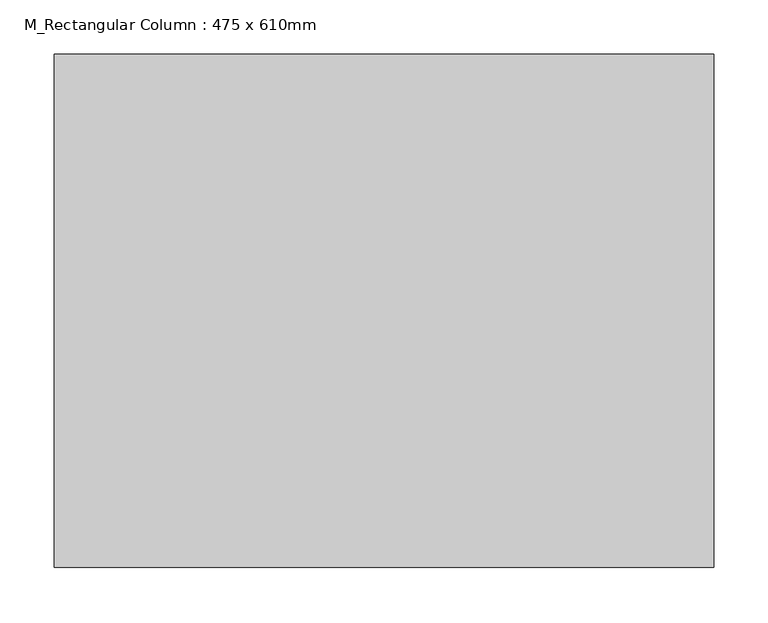
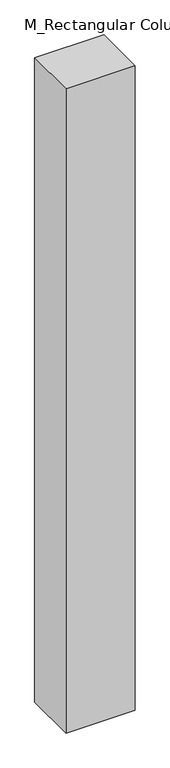
"""IFC4 building model written with IfcOpenShell, lengths in millimetres: column geometry, M_Rectangular Column : 475 x 610mm."""

from ifc_helpers import new_model, si_unit, origin, origin_with_axes, place, context, project, spatial, polyline, outline, extrude, source, transform, mapped, element, save


def m_rectangular_column_475_x_610mm_712a9979(model_context):
    return source(origin(), model_context, "Body", "SweptSolid", [
        extrude(outline(polyline([(305.0, 237.5), (305.0, -237.5), (-305.0, -237.5), (-305.0, 237.5), (305.0, 237.5)])), origin_with_axes(), (0.0, 0.0, 1.0), 6000.0),
    ])


if __name__ == "__main__":
    model = new_model("IFC4")
    model_context = context("Model", 3, world=origin())
    ifc_project = project(units=[si_unit("LENGTHUNIT", "METRE", prefix="MILLI")], contexts=[model_context])
    site = spatial("IfcSite", under=ifc_project)
    building = spatial("IfcBuilding", under=site)
    placement = place(None, origin())
    m_rectangular_column_475_x_610mm_shape = m_rectangular_column_475_x_610mm_712a9979(model_context)
    element("IfcColumn", 1, ObjectType="M_Rectangular Column : 475 x 610mm", at=placement, inside=building, context=model_context, shape_type="MappedRepresentation", body=[
        mapped(m_rectangular_column_475_x_610mm_shape, transform((0.0, 0.0, 0.0), x_axis=(1.0, 0.0, 0.0), y_axis=(0.0, 1.0, 0.0), z_axis=(0.0, 0.0, 1.0))),
    ])
    save(model, "model.ifc")

# Revit data of these elements
# Type "M_Rectangular Column : 475 x 610mm"
#   Depth = 475 mm
#   Offset Base = 0 mm
#   Offset Top = 0 mm
#   Width = 610 mm
#   Material = Copper
# Element 1 (IfcColumn, "M_Rectangular Column : 475 x 610mm")
#   Materials on its faces: "Copper"
# Materials
#   "Copper": class "Metal", colour RGB 0 0 0, transparency 0, Description = "Copper, matte finish", Cost = 0
